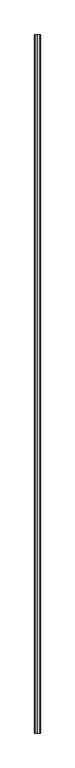
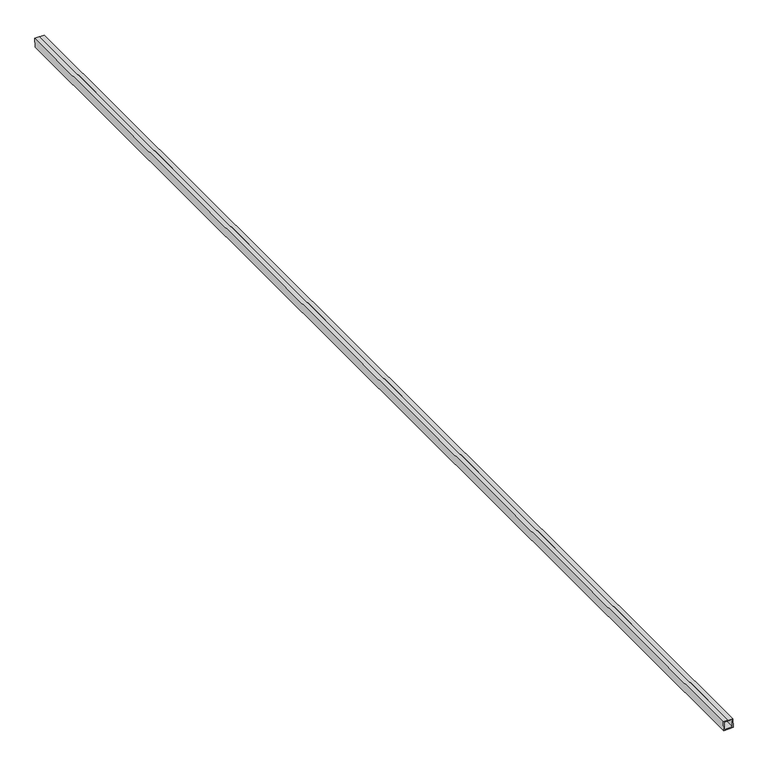
"""IFC4 building model written with IfcOpenShell, lengths in millimetres: proxy geometry, Inner panel:Inner panel:1:Inner panel:1 : Inner panel:Inner panel:300324:2:Inner panel:1:Inner panel:1 : Inner panel:Inner panel:300324:2 : Inner panel:Inner panel:1:Inner panel:1 : Inner panel:Inner panel:300324:300043:37 : Inner panel:Inner panel:1:Inner panel:1 : Inner panel:Inner panel:300324:2:Inner panel:1:Inner panel:1 : Inner panel:Inner panel:300324:2 : Inner panel:Inner panel:1:Inner panel:1 : Inner panel:Inner panel:300324:300043:308120."""

from ifc_helpers import new_model, si_unit, frame, origin, place, context, project, spatial, polyline, outline, extrude, source, transform, mapped, element, save


def generic_models_ada09204(model_context):
    return source(origin(), model_context, "Body", "SweptSolid", [
        extrude(outline(polyline([(4022.4868814, 562107.7864431), (4020.1076958, 562107.8855758), (4020.7685807, 562123.7468134), (3987.4599819, 562125.1346716), (3986.0721236, 562091.8260728), (4019.3807224, 562090.4382145), (4020.0416073, 562106.2994521), (4022.420793, 562106.2003193), (4021.6607753, 562087.9598962), (3983.5938052, 562089.5460199), (3985.179929, 562127.61299), (4023.2468991, 562126.0268663), (4022.4868814, 562107.7864431)])), frame((0.0, -575657.416384, 0.0), z_axis=(0.0, 1.0, 0.0), x_axis=(0.0, 0.0, 1.0)), (0.0, 0.0, 1.0), 4876.8),
    ])


if __name__ == "__main__":
    model = new_model("IFC4")
    model_context = context("Model", 3, world=origin())
    ifc_project = project(units=[si_unit("LENGTHUNIT", "METRE", prefix="MILLI")], contexts=[model_context])
    site = spatial("IfcSite", under=ifc_project)
    building = spatial("IfcBuilding", under=site)
    placement = place(None, origin())
    generic_models_shape = generic_models_ada09204(model_context)
    element("IfcBuildingElementProxy", 1, Name="Inner panel:Inner panel:1:Inner panel:1 : Inner panel:Inner panel:300324:2:Inner panel:1:Inner panel:1 : Inner panel:Inner panel:300324:2 : Inner panel:Inner panel:1:Inner panel:1 : Inner panel:Inner panel:300324:300043:37 : Inner panel:Inner panel:1:Inner panel:1 : Inner panel:Inner panel:300324:2:Inner panel:1:Inner panel:1 : Inner panel:Inner panel:300324:2 : Inner panel:Inner panel:1:Inner panel:1 : Inner panel:Inner panel:300324:300043:308120", ObjectType="Inner panel:Inner panel:1:Inner panel:1 : Inner panel:Inner panel:300324:2:Inner panel:1:Inner panel:1 : Inner panel:Inner panel:300324:2 : Inner panel:Inner panel:1:Inner panel:1 : Inner panel:Inner panel:300324:300043:37 : Inner panel:Inner panel:1:Inner panel:1 : Inner panel:Inner panel:300324:2:Inner panel:1:Inner panel:1 : Inner panel:Inner panel:300324:2 : Inner panel:Inner panel:1:Inner panel:1 : Inner panel:Inner panel:300324:300043:308120", at=placement, inside=building, context=model_context, shape_type="MappedRepresentation", body=[
        mapped(generic_models_shape, transform((0.0, 0.0, 0.0), x_axis=(1.0, 0.0, 0.0), y_axis=(0.0, 1.0, 0.0), z_axis=(0.0, 0.0, 1.0))),
    ])
    save(model, "model.ifc")

# Revit data of these elements
# Type "Inner panel:Inner panel:1:Inner panel:1 : Inner panel:Inner panel:300324:2:Inner panel:1:Inner panel:1 : Inner panel:Inner panel:300324:2 : Inner panel:Inner panel:1:Inner panel:1 : Inner panel:Inner panel:300324:300043:37 : Inner panel:Inner panel:1:Inner panel:1 : Inner panel:Inner panel:300324:2:Inner panel:1:Inner panel:1 : Inner panel:Inner panel:300324:2 : Inner panel:Inner panel:1:Inner panel:1 : Inner panel:Inner panel:300324:300043:308120"
#   NameOverride = "Inner panel:Inner panel:1:Inner panel:1 : Inner panel:Inner panel:300324:2:Inner panel:1:Inner panel:1 : Inner panel:Inner panel:300324:2 : Inner panel:Inner panel:1:Inner panel:1 : Inner panel:Inner panel:300324:300043:308120"
#   ObjectTypeOverride = "Inner panel:1:Inner panel:1 : Inner panel:Inner panel:300324:2 : Inner panel:Inner panel:1:Inner panel:1 : Inner panel:Inner panel:300324:300043"
#   Reference = "Inner panel"
#   Tag = "308120"
# Element 1 (IfcBuildingElementProxy, "Inner panel:Inner panel:1:Inner panel:1 : Inner panel:Inner panel:300324:2:Inner panel:1:Inner panel:1 : Inner panel:Inner panel:300324:2 : Inner panel:Inner panel:1:Inner panel:1 : Inner panel:Inner panel:300324:300043:37 : Inner panel:Inner panel:1:Inner panel:1 : Inner panel:Inner panel:300324:2:Inner panel:1:Inner panel:1 : Inner panel:Inner panel:300324:2 : Inner panel:Inner panel:1:Inner panel:1 : Inner panel:Inner panel:300324:300043:308120")
#   Materials on its faces: "1 1/2\" X 1 1/2\" x 1/8\" ALUM. TUBE (6061-T6) - (2) #16 WOOD SCREWS WITH 2.5\" EMBED AT EACH GLULAM - (1) SCREW AT ENDS"
# Materials
#   "1 1/2\" X 1 1/2\" x 1/8\" ALUM. TUBE (6061-T6) - (2) #16 WOOD SCREWS WITH 2.5\" EMBED AT EACH GLULAM - (1) SCREW AT ENDS": class "Unassigned", colour RGB 202 201 200, transparency 0, Cost = 0
